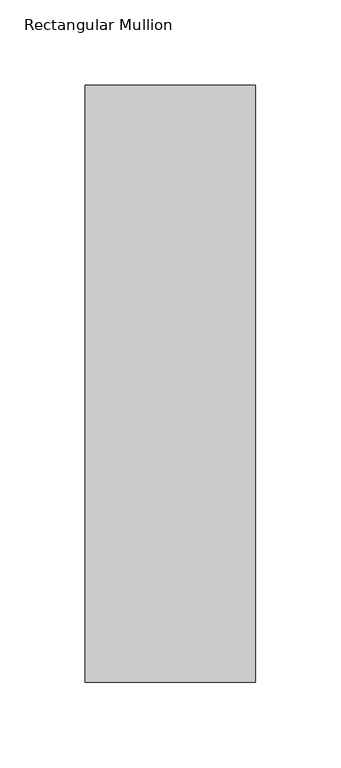
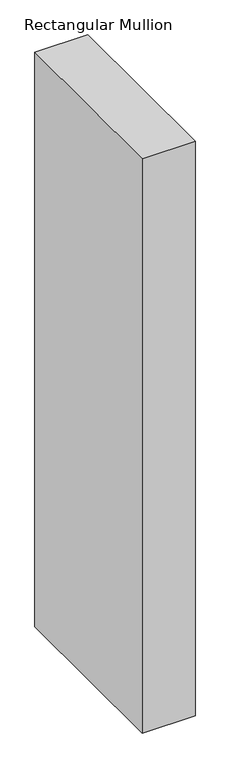
"""IFC4 building model written with IfcOpenShell, lengths in millimetres: member geometry, Rectangular Mullion : WWm-100x350-100mmOffset."""

import ifcopenshell
import ifcopenshell.guid

model = None  # the IFC model being written
_history = None  # IfcOwnerHistory: only IFC2X3 demands one
_inside = {}  # id of a spatial element -> (the spatial element, [elements in it])
_under = {}  # id of a project, library or spatial element -> (it, [spatial elements below it])
_declared = {}  # id of a project -> (the project, [libraries it declares])
_typed = {}  # id of a type object -> (the type object, [elements of that type])
_made_of = {}  # id of a material, layer set ... -> (it, [elements and type objects made of it])


def new_model(schema):
    """Start an empty IFC model of exactly this schema.

    Asked for "IFC4X3", IfcOpenShell would pick the latest addendum, in which some entities
    have other attributes; the version numbers below select the first issue.
    IFC2X3 requires an IfcOwnerHistory on every rooted entity: one is made here for all.
    """
    global model, _history
    if schema == "IFC4X3":
        model = ifcopenshell.file(schema_version=(4, 3, 0, 0))
    else:
        model = ifcopenshell.file(schema=schema)
    _inside.clear()
    _under.clear()
    _declared.clear()
    _typed.clear()
    _made_of.clear()
    _history = None
    if model.schema == "IFC2X3":
        org = make("IfcOrganization", Name="unknown")
        user = make(
            "IfcPersonAndOrganization",
            ThePerson=make("IfcPerson", FamilyName="unknown"),
            TheOrganization=org,
        )
        app = make(
            "IfcApplication",
            ApplicationDeveloper=org,
            Version="unknown",
            ApplicationFullName="unknown",
            ApplicationIdentifier="unknown",
        )
        _history = make(
            "IfcOwnerHistory",
            OwningUser=user,
            OwningApplication=app,
            ChangeAction="ADDED",
            CreationDate=0,
        )
    return model


def make(cls, **values):
    """One entity of the class cls with the attributes given. An attribute that is None is left unset."""
    return model.create_entity(
        cls, **{name: value for name, value in values.items() if value is not None}
    )


def rooted(cls, **values):
    """An entity with a GlobalId (a new one), such as an element, a storey or a relation."""
    return make(cls, GlobalId=ifcopenshell.guid.new(), OwnerHistory=_history, **values)


def si_unit(unit_type, name, prefix=None):
    """IfcSIUnit, for example si_unit("LENGTHUNIT", "METRE", prefix="MILLI")."""
    return make("IfcSIUnit", UnitType=unit_type, Prefix=prefix, Name=name)


def assignment(units):
    """IfcUnitAssignment: the units of a project."""
    return None if units is None else make("IfcUnitAssignment", Units=units)


def point(xyz):
    """IfcCartesianPoint."""
    return None if xyz is None else make("IfcCartesianPoint", Coordinates=xyz)


def direction(xyz):
    """IfcDirection."""
    return None if xyz is None else make("IfcDirection", DirectionRatios=xyz)


def frame(location, z_axis=None, x_axis=None):
    """IfcAxis2Placement3D, a coordinate frame: its origin and axes. An axis left out is left unset."""
    return make(
        "IfcAxis2Placement3D",
        Location=point(location),
        Axis=direction(z_axis),
        RefDirection=direction(x_axis),
    )


def origin():
    """The frame at (0, 0, 0) with its axes left unset."""
    return frame((0.0, 0.0, 0.0))


def place(relative_to, where):
    """IfcLocalPlacement: puts the frame where relative to a parent placement (None: the world)."""
    return make(
        "IfcLocalPlacement", PlacementRelTo=relative_to, RelativePlacement=where
    )


def context(
    kind, dimensions, precision=None, world=None, true_north=None, identifier=None
):
    """IfcGeometricRepresentationContext, for example the 3D "Model" context."""
    return make(
        "IfcGeometricRepresentationContext",
        ContextIdentifier=identifier,
        ContextType=kind,
        CoordinateSpaceDimension=dimensions,
        Precision=precision,
        WorldCoordinateSystem=world,
        TrueNorth=true_north,
    )


def project(units=None, contexts=None):
    """IfcProject with its units and contexts."""
    return rooted(
        "IfcProject",
        Name="project",
        RepresentationContexts=contexts,
        UnitsInContext=assignment(units),
    )


def spatial(cls, under=None, at=None, **own):
    """A site, building, storey or space (cls), placed at a placement, below another one or the project."""
    s = rooted(cls, ObjectPlacement=at, **own)
    if under is not None:
        _under.setdefault(under.id(), (under, []))[1].append(s)
    return s


def polyline(points):
    """IfcPolyline through the points."""
    return make("IfcPolyline", Points=[point(p) for p in points])


def outline(outer, holes=None, kind="AREA"):
    """IfcArbitraryClosedProfileDef: a profile drawn as a closed curve; with holes, ...WithVoids."""
    if holes is None:
        return make("IfcArbitraryClosedProfileDef", ProfileType=kind, OuterCurve=outer)
    return make(
        "IfcArbitraryProfileDefWithVoids",
        ProfileType=kind,
        OuterCurve=outer,
        InnerCurves=holes,
    )


def extrude(swept, where, along, depth):
    """IfcExtrudedAreaSolid: the profile swept, set in the frame where, extruded along a direction by depth."""
    return make(
        "IfcExtrudedAreaSolid",
        SweptArea=swept,
        Position=where,
        ExtrudedDirection=direction(along),
        Depth=depth,
    )


def shape(context_of_items, identifier, shape_type, items):
    """IfcShapeRepresentation: the items that make up one representation, for example the "Body"."""
    return make(
        "IfcShapeRepresentation",
        ContextOfItems=context_of_items,
        RepresentationIdentifier=identifier,
        RepresentationType=shape_type,
        Items=items,
    )


def source(mapping_origin, context_of_items, identifier, shape_type, items):
    """IfcRepresentationMap: a shape defined once, which mapped items show again and again."""
    return make(
        "IfcRepresentationMap",
        MappingOrigin=mapping_origin,
        MappedRepresentation=shape(context_of_items, identifier, shape_type, items),
    )


def transform(
    local_origin,
    x_axis=None,
    y_axis=None,
    z_axis=None,
    scale=None,
    scale2=None,
    scale3=None,
    uniform=True,
):
    """IfcCartesianTransformationOperator3D, or its non-uniform kind. x_axis, y_axis, z_axis: its Axis1, 2, 3."""
    if uniform:
        return make(
            "IfcCartesianTransformationOperator3D",
            Axis1=direction(x_axis),
            Axis2=direction(y_axis),
            LocalOrigin=point(local_origin),
            Scale=scale,
            Axis3=direction(z_axis),
        )
    return make(
        "IfcCartesianTransformationOperator3DnonUniform",
        Axis1=direction(x_axis),
        Axis2=direction(y_axis),
        LocalOrigin=point(local_origin),
        Scale=scale,
        Axis3=direction(z_axis),
        Scale2=scale2,
        Scale3=scale3,
    )


def mapped(mapping_source, mapping_target):
    """IfcMappedItem: shows the shape of a source again, moved by a transform."""
    return make(
        "IfcMappedItem", MappingSource=mapping_source, MappingTarget=mapping_target
    )


def made_of(thing, what):
    """Note that an element or type object is made of a material, layer set ...; save() writes the relation."""
    if what is not None:
        _made_of.setdefault(what.id(), (what, []))[1].append(thing)
    return thing


def element(
    cls,
    number,
    at=None,
    inside=None,
    cuts=None,
    type_object=None,
    material=None,
    context=None,
    identifier="Body",
    shape_type=None,
    held_by="IfcProductDefinitionShape",
    body=None,
    shapes=None,
    **own,
):
    """One element of the class cls, such as IfcWall. Its Tag is "e" and its number.

    at: its placement. inside: the storey or other place that contains it. cuts: it is an
    opening in that element (IfcRelVoidsElement). A single representation is given by context,
    identifier, shape_type and body (its items); several are given by shapes. held_by: the class
    of the entity that holds the representations. save() writes the other relations.
    """
    e = rooted(cls, Tag="e%d" % number, ObjectPlacement=at, **own)
    if body is not None:
        shapes = [shape(context, identifier, shape_type, body)]
    if shapes is not None:
        e.Representation = make(held_by, Representations=shapes)
    if inside is not None:
        _inside.setdefault(inside.id(), (inside, []))[1].append(e)
    if cuts is not None:
        rooted(
            "IfcRelVoidsElement", RelatingBuildingElement=cuts, RelatedOpeningElement=e
        )
    if type_object is not None:
        _typed.setdefault(type_object.id(), (type_object, []))[1].append(e)
    return made_of(e, material)


def aggregate(whole, parts):
    """IfcRelAggregates: a whole, such as a stair, and the parts it consists of."""
    return rooted("IfcRelAggregates", RelatingObject=whole, RelatedObjects=parts)


def save(model, path):
    """Write the relations noted so far, then the file.

    IfcRelAggregates (storeys below a building ...), IfcRelContainedInSpatialStructure (elements
    in a storey), IfcRelDefinesByType, IfcRelAssociatesMaterial and IfcRelDeclares: one each for
    every whole, place, type object, material and project.
    """
    for whole, parts in _under.values():
        aggregate(whole, parts)
    for where, things in _inside.values():
        rooted(
            "IfcRelContainedInSpatialStructure",
            RelatedElements=things,
            RelatingStructure=where,
        )
    for kind, things in _typed.values():
        rooted("IfcRelDefinesByType", RelatedObjects=things, RelatingType=kind)
    for what, things in _made_of.values():
        rooted("IfcRelAssociatesMaterial", RelatedObjects=things, RelatingMaterial=what)
    for by, libraries in _declared.values():
        rooted("IfcRelDeclares", RelatingContext=by, RelatedDefinitions=libraries)
    model.write(path)


def rectangular_mullion_8d887841(model_context):
    return source(origin(), model_context, "Body", "SweptSolid", [
        extrude(outline(polyline([(0.0, 175.0), (0.0, -175.0), (-100.0, -175.0), (-100.0, 175.0), (0.0, 175.0)])), frame((0.0, 0.0, -1145.1502132), z_axis=(0.0, 0.0, 1.0), x_axis=(1.0, 0.0, 0.0)), (0.0, 0.0, 1.0), 1145.1502132),
    ])


if __name__ == "__main__":
    model = new_model("IFC4")
    model_context = context("Model", 3, world=origin())
    ifc_project = project(units=[si_unit("LENGTHUNIT", "METRE", prefix="MILLI")], contexts=[model_context])
    site = spatial("IfcSite", under=ifc_project)
    building = spatial("IfcBuilding", under=site)
    placement = place(None, origin())
    rectangular_mullion_shape = rectangular_mullion_8d887841(model_context)
    element("IfcMember", 1, ObjectType="Rectangular Mullion : WWm-100x350-100mmOffset", at=placement, inside=building, context=model_context, shape_type="MappedRepresentation", body=[
        mapped(rectangular_mullion_shape, transform((0.0, 0.0, 0.0), x_axis=(1.0, 0.0, 0.0), y_axis=(0.0, 1.0, 0.0), z_axis=(0.0, 0.0, 1.0))),
    ])
    save(model, "model.ifc")

# Revit data of these elements
# Type "Rectangular Mullion : WWm-100x350-100mmOffset"
#   built-in parameter 1007304 = 1.14829 (stored number, unit not read)
#   built-in parameter 1007301 = 0.164042 (stored number, unit not read)
#   built-in parameter 1007300 = 0.164042 (stored number, unit not read)
# Element 1 (IfcMember, "Rectangular Mullion : WWm-100x350-100mmOffset")
#   Materials on its faces: "WW-EC-RGB-Mullion"
# Materials
#   "WW-EC-RGB-Mullion": class "Generic", colour RGB 255 255 255, transparency 0, Comments = "If region requests black mullions, switch asset color to RGB 25-25-25", Description = "Generic Color", Cost = 0
